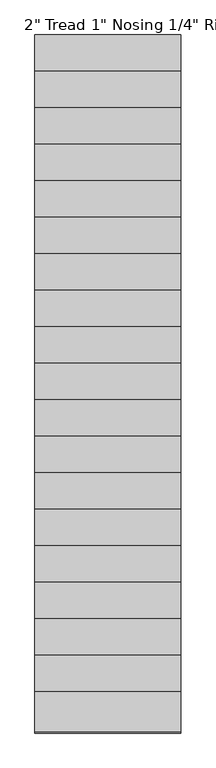
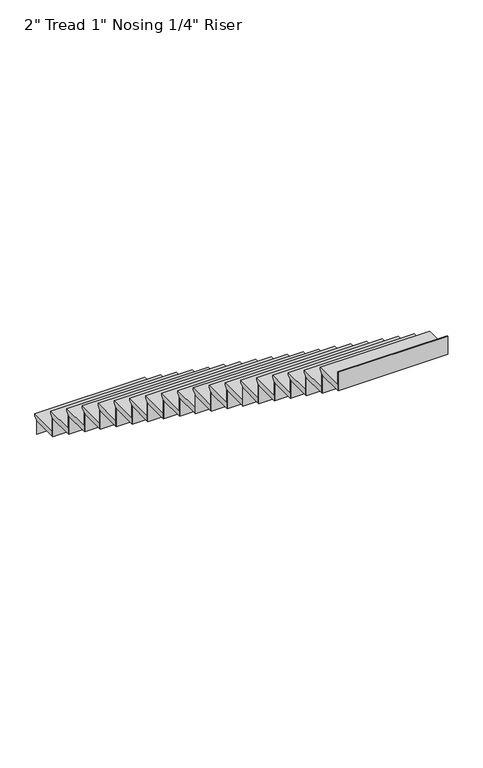
"""IFC4 building model written with IfcOpenShell, lengths in millimetres: stair flight geometry."""

import ifcopenshell
import ifcopenshell.guid

model = None  # the IFC model being written
_history = None  # IfcOwnerHistory: only IFC2X3 demands one
_inside = {}  # id of a spatial element -> (the spatial element, [elements in it])
_under = {}  # id of a project, library or spatial element -> (it, [spatial elements below it])
_declared = {}  # id of a project -> (the project, [libraries it declares])
_typed = {}  # id of a type object -> (the type object, [elements of that type])
_made_of = {}  # id of a material, layer set ... -> (it, [elements and type objects made of it])


def new_model(schema):
    """Start an empty IFC model of exactly this schema.

    Asked for "IFC4X3", IfcOpenShell would pick the latest addendum, in which some entities
    have other attributes; the version numbers below select the first issue.
    IFC2X3 requires an IfcOwnerHistory on every rooted entity: one is made here for all.
    """
    global model, _history
    if schema == "IFC4X3":
        model = ifcopenshell.file(schema_version=(4, 3, 0, 0))
    else:
        model = ifcopenshell.file(schema=schema)
    _inside.clear()
    _under.clear()
    _declared.clear()
    _typed.clear()
    _made_of.clear()
    _history = None
    if model.schema == "IFC2X3":
        org = make("IfcOrganization", Name="unknown")
        user = make(
            "IfcPersonAndOrganization",
            ThePerson=make("IfcPerson", FamilyName="unknown"),
            TheOrganization=org,
        )
        app = make(
            "IfcApplication",
            ApplicationDeveloper=org,
            Version="unknown",
            ApplicationFullName="unknown",
            ApplicationIdentifier="unknown",
        )
        _history = make(
            "IfcOwnerHistory",
            OwningUser=user,
            OwningApplication=app,
            ChangeAction="ADDED",
            CreationDate=0,
        )
    return model


def make(cls, **values):
    """One entity of the class cls with the attributes given. An attribute that is None is left unset."""
    return model.create_entity(
        cls, **{name: value for name, value in values.items() if value is not None}
    )


def rooted(cls, **values):
    """An entity with a GlobalId (a new one), such as an element, a storey or a relation."""
    return make(cls, GlobalId=ifcopenshell.guid.new(), OwnerHistory=_history, **values)


def si_unit(unit_type, name, prefix=None):
    """IfcSIUnit, for example si_unit("LENGTHUNIT", "METRE", prefix="MILLI")."""
    return make("IfcSIUnit", UnitType=unit_type, Prefix=prefix, Name=name)


def assignment(units):
    """IfcUnitAssignment: the units of a project."""
    return None if units is None else make("IfcUnitAssignment", Units=units)


def point(xyz):
    """IfcCartesianPoint."""
    return None if xyz is None else make("IfcCartesianPoint", Coordinates=xyz)


def direction(xyz):
    """IfcDirection."""
    return None if xyz is None else make("IfcDirection", DirectionRatios=xyz)


def frame(location, z_axis=None, x_axis=None):
    """IfcAxis2Placement3D, a coordinate frame: its origin and axes. An axis left out is left unset."""
    return make(
        "IfcAxis2Placement3D",
        Location=point(location),
        Axis=direction(z_axis),
        RefDirection=direction(x_axis),
    )


def origin():
    """The frame at (0, 0, 0) with its axes left unset."""
    return frame((0.0, 0.0, 0.0))


def origin_with_axes():
    """The frame at (0, 0, 0) with the z axis (0, 0, 1) and the x axis (1, 0, 0) written out."""
    return frame((0.0, 0.0, 0.0), z_axis=(0.0, 0.0, 1.0), x_axis=(1.0, 0.0, 0.0))


def place(relative_to, where):
    """IfcLocalPlacement: puts the frame where relative to a parent placement (None: the world)."""
    return make(
        "IfcLocalPlacement", PlacementRelTo=relative_to, RelativePlacement=where
    )


def context(
    kind, dimensions, precision=None, world=None, true_north=None, identifier=None
):
    """IfcGeometricRepresentationContext, for example the 3D "Model" context."""
    return make(
        "IfcGeometricRepresentationContext",
        ContextIdentifier=identifier,
        ContextType=kind,
        CoordinateSpaceDimension=dimensions,
        Precision=precision,
        WorldCoordinateSystem=world,
        TrueNorth=true_north,
    )


def project(units=None, contexts=None):
    """IfcProject with its units and contexts."""
    return rooted(
        "IfcProject",
        Name="project",
        RepresentationContexts=contexts,
        UnitsInContext=assignment(units),
    )


def spatial(cls, under=None, at=None, **own):
    """A site, building, storey or space (cls), placed at a placement, below another one or the project."""
    s = rooted(cls, ObjectPlacement=at, **own)
    if under is not None:
        _under.setdefault(under.id(), (under, []))[1].append(s)
    return s


def polyline(points):
    """IfcPolyline through the points."""
    return make("IfcPolyline", Points=[point(p) for p in points])


def outline(outer, holes=None, kind="AREA"):
    """IfcArbitraryClosedProfileDef: a profile drawn as a closed curve; with holes, ...WithVoids."""
    if holes is None:
        return make("IfcArbitraryClosedProfileDef", ProfileType=kind, OuterCurve=outer)
    return make(
        "IfcArbitraryProfileDefWithVoids",
        ProfileType=kind,
        OuterCurve=outer,
        InnerCurves=holes,
    )


def extrude(swept, where, along, depth):
    """IfcExtrudedAreaSolid: the profile swept, set in the frame where, extruded along a direction by depth."""
    return make(
        "IfcExtrudedAreaSolid",
        SweptArea=swept,
        Position=where,
        ExtrudedDirection=direction(along),
        Depth=depth,
    )


def shape(context_of_items, identifier, shape_type, items):
    """IfcShapeRepresentation: the items that make up one representation, for example the "Body"."""
    return make(
        "IfcShapeRepresentation",
        ContextOfItems=context_of_items,
        RepresentationIdentifier=identifier,
        RepresentationType=shape_type,
        Items=items,
    )


def source(mapping_origin, context_of_items, identifier, shape_type, items):
    """IfcRepresentationMap: a shape defined once, which mapped items show again and again."""
    return make(
        "IfcRepresentationMap",
        MappingOrigin=mapping_origin,
        MappedRepresentation=shape(context_of_items, identifier, shape_type, items),
    )


def transform(
    local_origin,
    x_axis=None,
    y_axis=None,
    z_axis=None,
    scale=None,
    scale2=None,
    scale3=None,
    uniform=True,
):
    """IfcCartesianTransformationOperator3D, or its non-uniform kind. x_axis, y_axis, z_axis: its Axis1, 2, 3."""
    if uniform:
        return make(
            "IfcCartesianTransformationOperator3D",
            Axis1=direction(x_axis),
            Axis2=direction(y_axis),
            LocalOrigin=point(local_origin),
            Scale=scale,
            Axis3=direction(z_axis),
        )
    return make(
        "IfcCartesianTransformationOperator3DnonUniform",
        Axis1=direction(x_axis),
        Axis2=direction(y_axis),
        LocalOrigin=point(local_origin),
        Scale=scale,
        Axis3=direction(z_axis),
        Scale2=scale2,
        Scale3=scale3,
    )


def mapped(mapping_source, mapping_target):
    """IfcMappedItem: shows the shape of a source again, moved by a transform."""
    return make(
        "IfcMappedItem", MappingSource=mapping_source, MappingTarget=mapping_target
    )


def made_of(thing, what):
    """Note that an element or type object is made of a material, layer set ...; save() writes the relation."""
    if what is not None:
        _made_of.setdefault(what.id(), (what, []))[1].append(thing)
    return thing


def element(
    cls,
    number,
    at=None,
    inside=None,
    cuts=None,
    type_object=None,
    material=None,
    context=None,
    identifier="Body",
    shape_type=None,
    held_by="IfcProductDefinitionShape",
    body=None,
    shapes=None,
    **own,
):
    """One element of the class cls, such as IfcWall. Its Tag is "e" and its number.

    at: its placement. inside: the storey or other place that contains it. cuts: it is an
    opening in that element (IfcRelVoidsElement). A single representation is given by context,
    identifier, shape_type and body (its items); several are given by shapes. held_by: the class
    of the entity that holds the representations. save() writes the other relations.
    """
    e = rooted(cls, Tag="e%d" % number, ObjectPlacement=at, **own)
    if body is not None:
        shapes = [shape(context, identifier, shape_type, body)]
    if shapes is not None:
        e.Representation = make(held_by, Representations=shapes)
    if inside is not None:
        _inside.setdefault(inside.id(), (inside, []))[1].append(e)
    if cuts is not None:
        rooted(
            "IfcRelVoidsElement", RelatingBuildingElement=cuts, RelatedOpeningElement=e
        )
    if type_object is not None:
        _typed.setdefault(type_object.id(), (type_object, []))[1].append(e)
    return made_of(e, material)


def aggregate(whole, parts):
    """IfcRelAggregates: a whole, such as a stair, and the parts it consists of."""
    return rooted("IfcRelAggregates", RelatingObject=whole, RelatedObjects=parts)


def save(model, path):
    """Write the relations noted so far, then the file.

    IfcRelAggregates (storeys below a building ...), IfcRelContainedInSpatialStructure (elements
    in a storey), IfcRelDefinesByType, IfcRelAssociatesMaterial and IfcRelDeclares: one each for
    every whole, place, type object, material and project.
    """
    for whole, parts in _under.values():
        aggregate(whole, parts)
    for where, things in _inside.values():
        rooted(
            "IfcRelContainedInSpatialStructure",
            RelatedElements=things,
            RelatingStructure=where,
        )
    for kind, things in _typed.values():
        rooted("IfcRelDefinesByType", RelatedObjects=things, RelatingType=kind)
    for what, things in _made_of.values():
        rooted("IfcRelAssociatesMaterial", RelatedObjects=things, RelatingMaterial=what)
    for by, libraries in _declared.values():
        rooted("IfcRelDeclares", RelatingContext=by, RelatedDefinitions=libraries)
    model.write(path)


def stair_flight_38837db3(model_context):
    return source(origin(), model_context, "Body", "SweptSolid", [
        extrude(outline(polyline([(-3242.0159434, 170.18), (-2975.3159434, 170.18), (-2975.3159434, 151.13), (-3000.7159434, 125.73), (-3000.7159434, 119.38), (-3242.0159434, 119.38), (-3242.0159434, 170.18)])), frame((31460.7652986, 0.0, 0.0), z_axis=(1.0, 0.0, 0.0), x_axis=(0.0, 1.0, 0.0)), (0.0, 0.0, 1.0), 965.2),
        extrude(outline(polyline([(31460.7652986, -3007.0659434), (31460.7652986, -3000.7159434), (32425.9652986, -3000.7159434), (32425.9652986, -3007.0659434), (31460.7652986, -3007.0659434)])), origin_with_axes(), (0.0, 0.0, 1.0), 119.38),
        extrude(outline(polyline([(31460.7652986, -3248.3659434), (31460.7652986, -3242.0159434), (32425.9652986, -3242.0159434), (32425.9652986, -3248.3659434), (31460.7652986, -3248.3659434)])), frame((0.0, 0.0, 119.38), z_axis=(0.0, 0.0, 1.0), x_axis=(1.0, 0.0, 0.0)), (0.0, 0.0, 1.0), 170.18),
        extrude(outline(polyline([(-3483.3159434, 340.36), (-3216.6159434, 340.36), (-3216.6159434, 321.31), (-3242.0159434, 295.91), (-3242.0159434, 289.56), (-3483.3159434, 289.56), (-3483.3159434, 340.36)])), frame((31460.7652986, 0.0, 0.0), z_axis=(1.0, 0.0, 0.0), x_axis=(0.0, 1.0, 0.0)), (0.0, 0.0, 1.0), 965.2),
        extrude(outline(polyline([(31460.7652986, -3489.6659434), (31460.7652986, -3483.3159434), (32425.9652986, -3483.3159434), (32425.9652986, -3489.6659434), (31460.7652986, -3489.6659434)])), frame((0.0, 0.0, 289.56), z_axis=(0.0, 0.0, 1.0), x_axis=(1.0, 0.0, 0.0)), (0.0, 0.0, 1.0), 170.18),
        extrude(outline(polyline([(-3724.6159434, 510.54), (-3457.9159434, 510.54), (-3457.9159434, 491.49), (-3483.3159434, 466.09), (-3483.3159434, 459.74), (-3724.6159434, 459.74), (-3724.6159434, 510.54)])), frame((31460.7652986, 0.0, 0.0), z_axis=(1.0, 0.0, 0.0), x_axis=(0.0, 1.0, 0.0)), (0.0, 0.0, 1.0), 965.2),
        extrude(outline(polyline([(31460.7652986, -3730.9659434), (31460.7652986, -3724.6159434), (32425.9652986, -3724.6159434), (32425.9652986, -3730.9659434), (31460.7652986, -3730.9659434)])), frame((0.0, 0.0, 459.74), z_axis=(0.0, 0.0, 1.0), x_axis=(1.0, 0.0, 0.0)), (0.0, 0.0, 1.0), 170.18),
        extrude(outline(polyline([(-3965.9159434, 680.72), (-3699.2159434, 680.72), (-3699.2159434, 661.67), (-3724.6159434, 636.27), (-3724.6159434, 629.92), (-3965.9159434, 629.92), (-3965.9159434, 680.72)])), frame((31460.7652986, 0.0, 0.0), z_axis=(1.0, 0.0, 0.0), x_axis=(0.0, 1.0, 0.0)), (0.0, 0.0, 1.0), 965.2),
        extrude(outline(polyline([(31460.7652986, -3972.2659434), (31460.7652986, -3965.9159434), (32425.9652986, -3965.9159434), (32425.9652986, -3972.2659434), (31460.7652986, -3972.2659434)])), frame((0.0, 0.0, 629.92), z_axis=(0.0, 0.0, 1.0), x_axis=(1.0, 0.0, 0.0)), (0.0, 0.0, 1.0), 170.18),
        extrude(outline(polyline([(-4207.2159434, 850.9), (-3940.5159434, 850.9), (-3940.5159434, 831.85), (-3965.9159434, 806.45), (-3965.9159434, 800.1), (-4207.2159434, 800.1), (-4207.2159434, 850.9)])), frame((31460.7652986, 0.0, 0.0), z_axis=(1.0, 0.0, 0.0), x_axis=(0.0, 1.0, 0.0)), (0.0, 0.0, 1.0), 965.2),
        extrude(outline(polyline([(31460.7652986, -4213.5659434), (31460.7652986, -4207.2159434), (32425.9652986, -4207.2159434), (32425.9652986, -4213.5659434), (31460.7652986, -4213.5659434)])), frame((0.0, 0.0, 800.1), z_axis=(0.0, 0.0, 1.0), x_axis=(1.0, 0.0, 0.0)), (0.0, 0.0, 1.0), 170.18),
        extrude(outline(polyline([(-4448.5159434, 1021.08), (-4181.8159434, 1021.08), (-4181.8159434, 1002.03), (-4207.2159434, 976.63), (-4207.2159434, 970.28), (-4448.5159434, 970.28), (-4448.5159434, 1021.08)])), frame((31460.7652986, 0.0, 0.0), z_axis=(1.0, 0.0, 0.0), x_axis=(0.0, 1.0, 0.0)), (0.0, 0.0, 1.0), 965.2),
        extrude(outline(polyline([(31460.7652986, -4454.8659434), (31460.7652986, -4448.5159434), (32425.9652986, -4448.5159434), (32425.9652986, -4454.8659434), (31460.7652986, -4454.8659434)])), frame((0.0, 0.0, 970.28), z_axis=(0.0, 0.0, 1.0), x_axis=(1.0, 0.0, 0.0)), (0.0, 0.0, 1.0), 170.18),
        extrude(outline(polyline([(-4689.8159434, 1191.26), (-4423.1159434, 1191.26), (-4423.1159434, 1172.21), (-4448.5159434, 1146.81), (-4448.5159434, 1140.46), (-4689.8159434, 1140.46), (-4689.8159434, 1191.26)])), frame((31460.7652986, 0.0, 0.0), z_axis=(1.0, 0.0, 0.0), x_axis=(0.0, 1.0, 0.0)), (0.0, 0.0, 1.0), 965.2),
        extrude(outline(polyline([(31460.7652986, -4696.1659434), (31460.7652986, -4689.8159434), (32425.9652986, -4689.8159434), (32425.9652986, -4696.1659434), (31460.7652986, -4696.1659434)])), frame((0.0, 0.0, 1140.46), z_axis=(0.0, 0.0, 1.0), x_axis=(1.0, 0.0, 0.0)), (0.0, 0.0, 1.0), 170.18),
        extrude(outline(polyline([(-4931.1159434, 1361.44), (-4664.4159434, 1361.44), (-4664.4159434, 1342.39), (-4689.8159434, 1316.99), (-4689.8159434, 1310.64), (-4931.1159434, 1310.64), (-4931.1159434, 1361.44)])), frame((31460.7652986, 0.0, 0.0), z_axis=(1.0, 0.0, 0.0), x_axis=(0.0, 1.0, 0.0)), (0.0, 0.0, 1.0), 965.2),
        extrude(outline(polyline([(31460.7652986, -4937.4659434), (31460.7652986, -4931.1159434), (32425.9652986, -4931.1159434), (32425.9652986, -4937.4659434), (31460.7652986, -4937.4659434)])), frame((0.0, 0.0, 1310.64), z_axis=(0.0, 0.0, 1.0), x_axis=(1.0, 0.0, 0.0)), (0.0, 0.0, 1.0), 170.18),
        extrude(outline(polyline([(-5172.4159434, 1531.62), (-4905.7159434, 1531.62), (-4905.7159434, 1512.57), (-4931.1159434, 1487.17), (-4931.1159434, 1480.82), (-5172.4159434, 1480.82), (-5172.4159434, 1531.62)])), frame((31460.7652986, 0.0, 0.0), z_axis=(1.0, 0.0, 0.0), x_axis=(0.0, 1.0, 0.0)), (0.0, 0.0, 1.0), 965.2),
        extrude(outline(polyline([(31460.7652986, -5178.7659434), (31460.7652986, -5172.4159434), (32425.9652986, -5172.4159434), (32425.9652986, -5178.7659434), (31460.7652986, -5178.7659434)])), frame((0.0, 0.0, 1480.82), z_axis=(0.0, 0.0, 1.0), x_axis=(1.0, 0.0, 0.0)), (0.0, 0.0, 1.0), 170.18),
        extrude(outline(polyline([(-5413.7159434, 1701.8), (-5147.0159434, 1701.8), (-5147.0159434, 1682.75), (-5172.4159434, 1657.35), (-5172.4159434, 1651.0), (-5413.7159434, 1651.0), (-5413.7159434, 1701.8)])), frame((31460.7652986, 0.0, 0.0), z_axis=(1.0, 0.0, 0.0), x_axis=(0.0, 1.0, 0.0)), (0.0, 0.0, 1.0), 965.2),
        extrude(outline(polyline([(31460.7652986, -5420.0659434), (31460.7652986, -5413.7159434), (32425.9652986, -5413.7159434), (32425.9652986, -5420.0659434), (31460.7652986, -5420.0659434)])), frame((0.0, 0.0, 1651.0), z_axis=(0.0, 0.0, 1.0), x_axis=(1.0, 0.0, 0.0)), (0.0, 0.0, 1.0), 170.18),
        extrude(outline(polyline([(-5655.0159434, 1871.98), (-5388.3159434, 1871.98), (-5388.3159434, 1852.93), (-5413.7159434, 1827.53), (-5413.7159434, 1821.18), (-5655.0159434, 1821.18), (-5655.0159434, 1871.98)])), frame((31460.7652986, 0.0, 0.0), z_axis=(1.0, 0.0, 0.0), x_axis=(0.0, 1.0, 0.0)), (0.0, 0.0, 1.0), 965.2),
        extrude(outline(polyline([(31460.7652986, -5661.3659434), (31460.7652986, -5655.0159434), (32425.9652986, -5655.0159434), (32425.9652986, -5661.3659434), (31460.7652986, -5661.3659434)])), frame((0.0, 0.0, 1821.18), z_axis=(0.0, 0.0, 1.0), x_axis=(1.0, 0.0, 0.0)), (0.0, 0.0, 1.0), 170.18),
        extrude(outline(polyline([(-5896.3159434, 2042.16), (-5629.6159434, 2042.16), (-5629.6159434, 2023.11), (-5655.0159434, 1997.71), (-5655.0159434, 1991.36), (-5896.3159434, 1991.36), (-5896.3159434, 2042.16)])), frame((31460.7652986, 0.0, 0.0), z_axis=(1.0, 0.0, 0.0), x_axis=(0.0, 1.0, 0.0)), (0.0, 0.0, 1.0), 965.2),
        extrude(outline(polyline([(31460.7652986, -5902.6659434), (31460.7652986, -5896.3159434), (32425.9652986, -5896.3159434), (32425.9652986, -5902.6659434), (31460.7652986, -5902.6659434)])), frame((0.0, 0.0, 1991.36), z_axis=(0.0, 0.0, 1.0), x_axis=(1.0, 0.0, 0.0)), (0.0, 0.0, 1.0), 170.18),
        extrude(outline(polyline([(-6137.6159434, 2212.34), (-5870.9159434, 2212.34), (-5870.9159434, 2193.29), (-5896.3159434, 2167.89), (-5896.3159434, 2161.54), (-6137.6159434, 2161.54), (-6137.6159434, 2212.34)])), frame((31460.7652986, 0.0, 0.0), z_axis=(1.0, 0.0, 0.0), x_axis=(0.0, 1.0, 0.0)), (0.0, 0.0, 1.0), 965.2),
        extrude(outline(polyline([(31460.7652986, -6143.9659434), (31460.7652986, -6137.6159434), (32425.9652986, -6137.6159434), (32425.9652986, -6143.9659434), (31460.7652986, -6143.9659434)])), frame((0.0, 0.0, 2161.54), z_axis=(0.0, 0.0, 1.0), x_axis=(1.0, 0.0, 0.0)), (0.0, 0.0, 1.0), 170.18),
        extrude(outline(polyline([(-6378.9159434, 2382.52), (-6112.2159434, 2382.52), (-6112.2159434, 2363.47), (-6137.6159434, 2338.07), (-6137.6159434, 2331.72), (-6378.9159434, 2331.72), (-6378.9159434, 2382.52)])), frame((31460.7652986, 0.0, 0.0), z_axis=(1.0, 0.0, 0.0), x_axis=(0.0, 1.0, 0.0)), (0.0, 0.0, 1.0), 965.2),
        extrude(outline(polyline([(31460.7652986, -6385.2659434), (31460.7652986, -6378.9159434), (32425.9652986, -6378.9159434), (32425.9652986, -6385.2659434), (31460.7652986, -6385.2659434)])), frame((0.0, 0.0, 2331.72), z_axis=(0.0, 0.0, 1.0), x_axis=(1.0, 0.0, 0.0)), (0.0, 0.0, 1.0), 170.18),
        extrude(outline(polyline([(-6620.2159434, 2552.7), (-6353.5159434, 2552.7), (-6353.5159434, 2533.65), (-6378.9159434, 2508.25), (-6378.9159434, 2501.9), (-6620.2159434, 2501.9), (-6620.2159434, 2552.7)])), frame((31460.7652986, 0.0, 0.0), z_axis=(1.0, 0.0, 0.0), x_axis=(0.0, 1.0, 0.0)), (0.0, 0.0, 1.0), 965.2),
        extrude(outline(polyline([(31460.7652986, -6626.5659434), (31460.7652986, -6620.2159434), (32425.9652986, -6620.2159434), (32425.9652986, -6626.5659434), (31460.7652986, -6626.5659434)])), frame((0.0, 0.0, 2501.9), z_axis=(0.0, 0.0, 1.0), x_axis=(1.0, 0.0, 0.0)), (0.0, 0.0, 1.0), 170.18),
        extrude(outline(polyline([(-6861.5159434, 2722.88), (-6594.8159434, 2722.88), (-6594.8159434, 2703.83), (-6620.2159434, 2678.43), (-6620.2159434, 2672.08), (-6861.5159434, 2672.08), (-6861.5159434, 2722.88)])), frame((31460.7652986, 0.0, 0.0), z_axis=(1.0, 0.0, 0.0), x_axis=(0.0, 1.0, 0.0)), (0.0, 0.0, 1.0), 965.2),
        extrude(outline(polyline([(31460.7652986, -6867.8659434), (31460.7652986, -6861.5159434), (32425.9652986, -6861.5159434), (32425.9652986, -6867.8659434), (31460.7652986, -6867.8659434)])), frame((0.0, 0.0, 2672.08), z_axis=(0.0, 0.0, 1.0), x_axis=(1.0, 0.0, 0.0)), (0.0, 0.0, 1.0), 170.18),
        extrude(outline(polyline([(-7102.8159434, 2893.06), (-6836.1159434, 2893.06), (-6836.1159434, 2874.01), (-6861.5159434, 2848.61), (-6861.5159434, 2842.26), (-7102.8159434, 2842.26), (-7102.8159434, 2893.06)])), frame((31460.7652986, 0.0, 0.0), z_axis=(1.0, 0.0, 0.0), x_axis=(0.0, 1.0, 0.0)), (0.0, 0.0, 1.0), 965.2),
        extrude(outline(polyline([(31460.7652986, -7109.1659434), (31460.7652986, -7102.8159434), (32425.9652986, -7102.8159434), (32425.9652986, -7109.1659434), (31460.7652986, -7109.1659434)])), frame((0.0, 0.0, 2842.26), z_axis=(0.0, 0.0, 1.0), x_axis=(1.0, 0.0, 0.0)), (0.0, 0.0, 1.0), 170.18),
        extrude(outline(polyline([(-7344.1159434, 3063.24), (-7077.4159434, 3063.24), (-7077.4159434, 3044.19), (-7102.8159434, 3018.79), (-7102.8159434, 3012.44), (-7344.1159434, 3012.44), (-7344.1159434, 3063.24)])), frame((31460.7652986, 0.0, 0.0), z_axis=(1.0, 0.0, 0.0), x_axis=(0.0, 1.0, 0.0)), (0.0, 0.0, 1.0), 965.2),
        extrude(outline(polyline([(31460.7652986, -7350.4659434), (31460.7652986, -7344.1159434), (32425.9652986, -7344.1159434), (32425.9652986, -7350.4659434), (31460.7652986, -7350.4659434)])), frame((0.0, 0.0, 3012.44), z_axis=(0.0, 0.0, 1.0), x_axis=(1.0, 0.0, 0.0)), (0.0, 0.0, 1.0), 170.18),
        extrude(outline(polyline([(-7585.4159434, 3233.42), (-7318.7159434, 3233.42), (-7318.7159434, 3214.37), (-7344.1159434, 3188.97), (-7344.1159434, 3182.62), (-7585.4159434, 3182.62), (-7585.4159434, 3233.42)])), frame((31460.7652986, 0.0, 0.0), z_axis=(1.0, 0.0, 0.0), x_axis=(0.0, 1.0, 0.0)), (0.0, 0.0, 1.0), 965.2),
        extrude(outline(polyline([(31460.7652986, -7591.7659434), (31460.7652986, -7585.4159434), (32425.9652986, -7585.4159434), (32425.9652986, -7591.7659434), (31460.7652986, -7591.7659434)])), frame((0.0, 0.0, 3182.62), z_axis=(0.0, 0.0, 1.0), x_axis=(1.0, 0.0, 0.0)), (0.0, 0.0, 1.0), 170.18),
    ])


if __name__ == "__main__":
    model = new_model("IFC4")
    model_context = context("Model", 3, world=origin())
    ifc_project = project(units=[si_unit("LENGTHUNIT", "METRE", prefix="MILLI")], contexts=[model_context])
    site = spatial("IfcSite", under=ifc_project)
    building = spatial("IfcBuilding", under=site)
    placement = place(None, origin())
    stair_flight_shape = stair_flight_38837db3(model_context)
    element("IfcStairFlight", 1, ObjectType="2\" Tread 1\" Nosing 1/4\" Riser", at=placement, inside=building, context=model_context, shape_type="MappedRepresentation", body=[
        mapped(stair_flight_shape, transform((0.0, 0.0, 0.0), x_axis=(1.0, 0.0, 0.0), y_axis=(0.0, 1.0, 0.0), z_axis=(0.0, 0.0, 1.0))),
    ])
    save(model, "model.ifc")

# Revit data of these elements
# Element 1 (IfcStairFlight, "2\" Tread 1\" Nosing 1/4\" Riser")
#   Materials on its faces: "Default Floor"
# Materials
#   "Default Floor": class "Miscellaneous", colour RGB 255 255 255, transparency 0, Cost = 0
